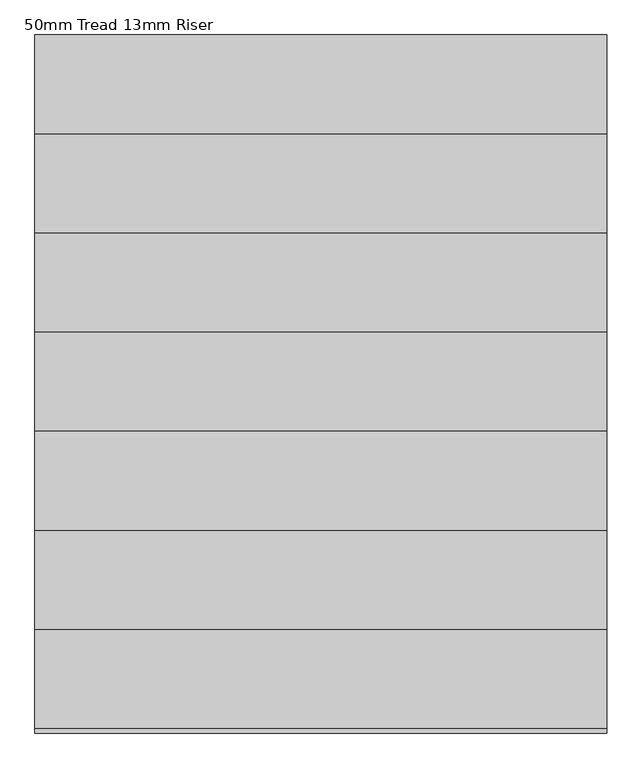
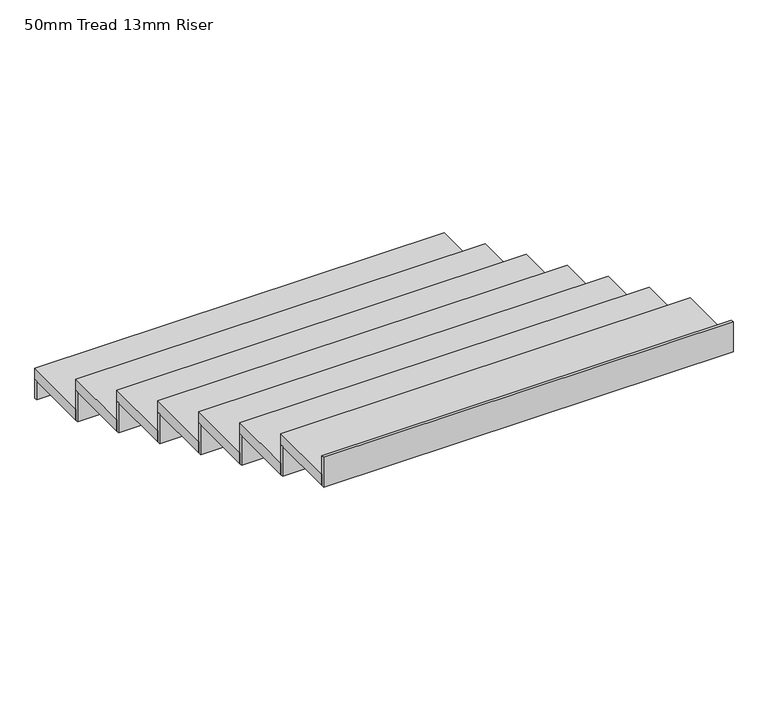
"""IFC4 building model written with IfcOpenShell, lengths in millimetres: stair flight geometry, 50mm Tread 13mm Riser."""

import ifcopenshell
import ifcopenshell.guid

model = None  # the IFC model being written
_history = None  # IfcOwnerHistory: only IFC2X3 demands one
_inside = {}  # id of a spatial element -> (the spatial element, [elements in it])
_under = {}  # id of a project, library or spatial element -> (it, [spatial elements below it])
_declared = {}  # id of a project -> (the project, [libraries it declares])
_typed = {}  # id of a type object -> (the type object, [elements of that type])
_made_of = {}  # id of a material, layer set ... -> (it, [elements and type objects made of it])


def new_model(schema):
    """Start an empty IFC model of exactly this schema.

    Asked for "IFC4X3", IfcOpenShell would pick the latest addendum, in which some entities
    have other attributes; the version numbers below select the first issue.
    IFC2X3 requires an IfcOwnerHistory on every rooted entity: one is made here for all.
    """
    global model, _history
    if schema == "IFC4X3":
        model = ifcopenshell.file(schema_version=(4, 3, 0, 0))
    else:
        model = ifcopenshell.file(schema=schema)
    _inside.clear()
    _under.clear()
    _declared.clear()
    _typed.clear()
    _made_of.clear()
    _history = None
    if model.schema == "IFC2X3":
        org = make("IfcOrganization", Name="unknown")
        user = make(
            "IfcPersonAndOrganization",
            ThePerson=make("IfcPerson", FamilyName="unknown"),
            TheOrganization=org,
        )
        app = make(
            "IfcApplication",
            ApplicationDeveloper=org,
            Version="unknown",
            ApplicationFullName="unknown",
            ApplicationIdentifier="unknown",
        )
        _history = make(
            "IfcOwnerHistory",
            OwningUser=user,
            OwningApplication=app,
            ChangeAction="ADDED",
            CreationDate=0,
        )
    return model


def make(cls, **values):
    """One entity of the class cls with the attributes given. An attribute that is None is left unset."""
    return model.create_entity(
        cls, **{name: value for name, value in values.items() if value is not None}
    )


def rooted(cls, **values):
    """An entity with a GlobalId (a new one), such as an element, a storey or a relation."""
    return make(cls, GlobalId=ifcopenshell.guid.new(), OwnerHistory=_history, **values)


def si_unit(unit_type, name, prefix=None):
    """IfcSIUnit, for example si_unit("LENGTHUNIT", "METRE", prefix="MILLI")."""
    return make("IfcSIUnit", UnitType=unit_type, Prefix=prefix, Name=name)


def assignment(units):
    """IfcUnitAssignment: the units of a project."""
    return None if units is None else make("IfcUnitAssignment", Units=units)


def point(xyz):
    """IfcCartesianPoint."""
    return None if xyz is None else make("IfcCartesianPoint", Coordinates=xyz)


def direction(xyz):
    """IfcDirection."""
    return None if xyz is None else make("IfcDirection", DirectionRatios=xyz)


def frame(location, z_axis=None, x_axis=None):
    """IfcAxis2Placement3D, a coordinate frame: its origin and axes. An axis left out is left unset."""
    return make(
        "IfcAxis2Placement3D",
        Location=point(location),
        Axis=direction(z_axis),
        RefDirection=direction(x_axis),
    )


def origin():
    """The frame at (0, 0, 0) with its axes left unset."""
    return frame((0.0, 0.0, 0.0))


def place(relative_to, where):
    """IfcLocalPlacement: puts the frame where relative to a parent placement (None: the world)."""
    return make(
        "IfcLocalPlacement", PlacementRelTo=relative_to, RelativePlacement=where
    )


def context(
    kind, dimensions, precision=None, world=None, true_north=None, identifier=None
):
    """IfcGeometricRepresentationContext, for example the 3D "Model" context."""
    return make(
        "IfcGeometricRepresentationContext",
        ContextIdentifier=identifier,
        ContextType=kind,
        CoordinateSpaceDimension=dimensions,
        Precision=precision,
        WorldCoordinateSystem=world,
        TrueNorth=true_north,
    )


def project(units=None, contexts=None):
    """IfcProject with its units and contexts."""
    return rooted(
        "IfcProject",
        Name="project",
        RepresentationContexts=contexts,
        UnitsInContext=assignment(units),
    )


def spatial(cls, under=None, at=None, **own):
    """A site, building, storey or space (cls), placed at a placement, below another one or the project."""
    s = rooted(cls, ObjectPlacement=at, **own)
    if under is not None:
        _under.setdefault(under.id(), (under, []))[1].append(s)
    return s


def polyline(points):
    """IfcPolyline through the points."""
    return make("IfcPolyline", Points=[point(p) for p in points])


def outline(outer, holes=None, kind="AREA"):
    """IfcArbitraryClosedProfileDef: a profile drawn as a closed curve; with holes, ...WithVoids."""
    if holes is None:
        return make("IfcArbitraryClosedProfileDef", ProfileType=kind, OuterCurve=outer)
    return make(
        "IfcArbitraryProfileDefWithVoids",
        ProfileType=kind,
        OuterCurve=outer,
        InnerCurves=holes,
    )


def extrude(swept, where, along, depth):
    """IfcExtrudedAreaSolid: the profile swept, set in the frame where, extruded along a direction by depth."""
    return make(
        "IfcExtrudedAreaSolid",
        SweptArea=swept,
        Position=where,
        ExtrudedDirection=direction(along),
        Depth=depth,
    )


def shape(context_of_items, identifier, shape_type, items):
    """IfcShapeRepresentation: the items that make up one representation, for example the "Body"."""
    return make(
        "IfcShapeRepresentation",
        ContextOfItems=context_of_items,
        RepresentationIdentifier=identifier,
        RepresentationType=shape_type,
        Items=items,
    )


def source(mapping_origin, context_of_items, identifier, shape_type, items):
    """IfcRepresentationMap: a shape defined once, which mapped items show again and again."""
    return make(
        "IfcRepresentationMap",
        MappingOrigin=mapping_origin,
        MappedRepresentation=shape(context_of_items, identifier, shape_type, items),
    )


def transform(
    local_origin,
    x_axis=None,
    y_axis=None,
    z_axis=None,
    scale=None,
    scale2=None,
    scale3=None,
    uniform=True,
):
    """IfcCartesianTransformationOperator3D, or its non-uniform kind. x_axis, y_axis, z_axis: its Axis1, 2, 3."""
    if uniform:
        return make(
            "IfcCartesianTransformationOperator3D",
            Axis1=direction(x_axis),
            Axis2=direction(y_axis),
            LocalOrigin=point(local_origin),
            Scale=scale,
            Axis3=direction(z_axis),
        )
    return make(
        "IfcCartesianTransformationOperator3DnonUniform",
        Axis1=direction(x_axis),
        Axis2=direction(y_axis),
        LocalOrigin=point(local_origin),
        Scale=scale,
        Axis3=direction(z_axis),
        Scale2=scale2,
        Scale3=scale3,
    )


def mapped(mapping_source, mapping_target):
    """IfcMappedItem: shows the shape of a source again, moved by a transform."""
    return make(
        "IfcMappedItem", MappingSource=mapping_source, MappingTarget=mapping_target
    )


def made_of(thing, what):
    """Note that an element or type object is made of a material, layer set ...; save() writes the relation."""
    if what is not None:
        _made_of.setdefault(what.id(), (what, []))[1].append(thing)
    return thing


def element(
    cls,
    number,
    at=None,
    inside=None,
    cuts=None,
    type_object=None,
    material=None,
    context=None,
    identifier="Body",
    shape_type=None,
    held_by="IfcProductDefinitionShape",
    body=None,
    shapes=None,
    **own,
):
    """One element of the class cls, such as IfcWall. Its Tag is "e" and its number.

    at: its placement. inside: the storey or other place that contains it. cuts: it is an
    opening in that element (IfcRelVoidsElement). A single representation is given by context,
    identifier, shape_type and body (its items); several are given by shapes. held_by: the class
    of the entity that holds the representations. save() writes the other relations.
    """
    e = rooted(cls, Tag="e%d" % number, ObjectPlacement=at, **own)
    if body is not None:
        shapes = [shape(context, identifier, shape_type, body)]
    if shapes is not None:
        e.Representation = make(held_by, Representations=shapes)
    if inside is not None:
        _inside.setdefault(inside.id(), (inside, []))[1].append(e)
    if cuts is not None:
        rooted(
            "IfcRelVoidsElement", RelatingBuildingElement=cuts, RelatedOpeningElement=e
        )
    if type_object is not None:
        _typed.setdefault(type_object.id(), (type_object, []))[1].append(e)
    return made_of(e, material)


def aggregate(whole, parts):
    """IfcRelAggregates: a whole, such as a stair, and the parts it consists of."""
    return rooted("IfcRelAggregates", RelatingObject=whole, RelatedObjects=parts)


def save(model, path):
    """Write the relations noted so far, then the file.

    IfcRelAggregates (storeys below a building ...), IfcRelContainedInSpatialStructure (elements
    in a storey), IfcRelDefinesByType, IfcRelAssociatesMaterial and IfcRelDeclares: one each for
    every whole, place, type object, material and project.
    """
    for whole, parts in _under.values():
        aggregate(whole, parts)
    for where, things in _inside.values():
        rooted(
            "IfcRelContainedInSpatialStructure",
            RelatedElements=things,
            RelatingStructure=where,
        )
    for kind, things in _typed.values():
        rooted("IfcRelDefinesByType", RelatedObjects=things, RelatingType=kind)
    for what, things in _made_of.values():
        rooted("IfcRelAssociatesMaterial", RelatedObjects=things, RelatingMaterial=what)
    for by, libraries in _declared.values():
        rooted("IfcRelDeclares", RelatingContext=by, RelatedDefinitions=libraries)
    model.write(path)


def stair_flight_50mm_tread_13mm_riser_d40b31cd(model_context):
    return source(origin(), model_context, "Body", "SweptSolid", [
        extrude(outline(polyline([(-13215.2814495, -5630.5731037), (-13215.2814495, -5618.0731037), (-11485.2814495, -5618.0731037), (-11485.2814495, -5630.5731037), (-13215.2814495, -5630.5731037)])), frame((0.0, 0.0, -1066.6666667), z_axis=(0.0, 0.0, 1.0), x_axis=(1.0, 0.0, 0.0)), (0.0, 0.0, 1.0), 83.3333333),
        extrude(outline(polyline([(-11485.2814495, -5918.0731037), (-13215.2814495, -5918.0731037), (-13215.2814495, -5618.0731037), (-11485.2814495, -5618.0731037), (-11485.2814495, -5918.0731037)])), frame((0.0, 0.0, -983.3333333), z_axis=(0.0, 0.0, 1.0), x_axis=(1.0, 0.0, 0.0)), (0.0, 0.0, 1.0), 50.0),
        extrude(outline(polyline([(-13215.2814495, -5930.5731037), (-13215.2814495, -5918.0731037), (-11485.2814495, -5918.0731037), (-11485.2814495, -5930.5731037), (-13215.2814495, -5930.5731037)])), frame((0.0, 0.0, -983.3333333), z_axis=(0.0, 0.0, 1.0), x_axis=(1.0, 0.0, 0.0)), (0.0, 0.0, 1.0), 133.3333333),
        extrude(outline(polyline([(-11485.2814495, -6218.0731037), (-13215.2814495, -6218.0731037), (-13215.2814495, -5918.0731037), (-11485.2814495, -5918.0731037), (-11485.2814495, -6218.0731037)])), frame((0.0, 0.0, -850.0), z_axis=(0.0, 0.0, 1.0), x_axis=(1.0, 0.0, 0.0)), (0.0, 0.0, 1.0), 50.0),
        extrude(outline(polyline([(-13215.2814495, -6230.5731037), (-13215.2814495, -6218.0731037), (-11485.2814495, -6218.0731037), (-11485.2814495, -6230.5731037), (-13215.2814495, -6230.5731037)])), frame((0.0, 0.0, -850.0), z_axis=(0.0, 0.0, 1.0), x_axis=(1.0, 0.0, 0.0)), (0.0, 0.0, 1.0), 133.3333333),
        extrude(outline(polyline([(-11485.2814495, -6518.0731037), (-13215.2814495, -6518.0731037), (-13215.2814495, -6218.0731037), (-11485.2814495, -6218.0731037), (-11485.2814495, -6518.0731037)])), frame((0.0, 0.0, -716.6666667), z_axis=(0.0, 0.0, 1.0), x_axis=(1.0, 0.0, 0.0)), (0.0, 0.0, 1.0), 50.0),
        extrude(outline(polyline([(-13215.2814495, -6530.5731037), (-13215.2814495, -6518.0731037), (-11485.2814495, -6518.0731037), (-11485.2814495, -6530.5731037), (-13215.2814495, -6530.5731037)])), frame((0.0, 0.0, -716.6666667), z_axis=(0.0, 0.0, 1.0), x_axis=(1.0, 0.0, 0.0)), (0.0, 0.0, 1.0), 133.3333333),
        extrude(outline(polyline([(-11485.2814495, -6818.0731037), (-13215.2814495, -6818.0731037), (-13215.2814495, -6518.0731037), (-11485.2814495, -6518.0731037), (-11485.2814495, -6818.0731037)])), frame((0.0, 0.0, -583.3333333), z_axis=(0.0, 0.0, 1.0), x_axis=(1.0, 0.0, 0.0)), (0.0, 0.0, 1.0), 50.0),
        extrude(outline(polyline([(-13215.2814495, -6830.5731037), (-13215.2814495, -6818.0731037), (-11485.2814495, -6818.0731037), (-11485.2814495, -6830.5731037), (-13215.2814495, -6830.5731037)])), frame((0.0, 0.0, -583.3333333), z_axis=(0.0, 0.0, 1.0), x_axis=(1.0, 0.0, 0.0)), (0.0, 0.0, 1.0), 133.3333333),
        extrude(outline(polyline([(-11485.2814495, -7118.0731037), (-13215.2814495, -7118.0731037), (-13215.2814495, -6818.0731037), (-11485.2814495, -6818.0731037), (-11485.2814495, -7118.0731037)])), frame((0.0, 0.0, -450.0), z_axis=(0.0, 0.0, 1.0), x_axis=(1.0, 0.0, 0.0)), (0.0, 0.0, 1.0), 50.0),
        extrude(outline(polyline([(-13215.2814495, -7130.5731037), (-13215.2814495, -7118.0731037), (-11485.2814495, -7118.0731037), (-11485.2814495, -7130.5731037), (-13215.2814495, -7130.5731037)])), frame((0.0, 0.0, -450.0), z_axis=(0.0, 0.0, 1.0), x_axis=(1.0, 0.0, 0.0)), (0.0, 0.0, 1.0), 133.3333333),
        extrude(outline(polyline([(-11485.2814495, -7418.0731037), (-13215.2814495, -7418.0731037), (-13215.2814495, -7118.0731037), (-11485.2814495, -7118.0731037), (-11485.2814495, -7418.0731037)])), frame((0.0, 0.0, -316.6666667), z_axis=(0.0, 0.0, 1.0), x_axis=(1.0, 0.0, 0.0)), (0.0, 0.0, 1.0), 50.0),
        extrude(outline(polyline([(-13215.2814495, -7430.5731037), (-13215.2814495, -7418.0731037), (-11485.2814495, -7418.0731037), (-11485.2814495, -7430.5731037), (-13215.2814495, -7430.5731037)])), frame((0.0, 0.0, -316.6666667), z_axis=(0.0, 0.0, 1.0), x_axis=(1.0, 0.0, 0.0)), (0.0, 0.0, 1.0), 133.3333333),
        extrude(outline(polyline([(-13215.2814495, -7730.5731037), (-13215.2814495, -7718.0731037), (-11485.2814495, -7718.0731037), (-11485.2814495, -7730.5731037), (-13215.2814495, -7730.5731037)])), frame((0.0, 0.0, -183.3333333), z_axis=(0.0, 0.0, 1.0), x_axis=(1.0, 0.0, 0.0)), (0.0, 0.0, 1.0), 133.3333333),
        extrude(outline(polyline([(-11485.2814495, -7718.0731037), (-13215.2814495, -7718.0731037), (-13215.2814495, -7418.0731037), (-11485.2814495, -7418.0731037), (-11485.2814495, -7718.0731037)])), frame((0.0, 0.0, -183.3333333), z_axis=(0.0, 0.0, 1.0), x_axis=(1.0, 0.0, 0.0)), (0.0, 0.0, 1.0), 50.0),
    ])


if __name__ == "__main__":
    model = new_model("IFC4")
    model_context = context("Model", 3, world=origin())
    ifc_project = project(units=[si_unit("LENGTHUNIT", "METRE", prefix="MILLI")], contexts=[model_context])
    site = spatial("IfcSite", under=ifc_project)
    building = spatial("IfcBuilding", under=site)
    placement = place(None, origin())
    stair_flight_50mm_tread_13mm_riser_shape = stair_flight_50mm_tread_13mm_riser_d40b31cd(model_context)
    element("IfcStairFlight", 1, ObjectType="50mm Tread 13mm Riser", at=placement, inside=building, context=model_context, shape_type="MappedRepresentation", body=[
        mapped(stair_flight_50mm_tread_13mm_riser_shape, transform((0.0, 0.0, 0.0), x_axis=(1.0, 0.0, 0.0), y_axis=(0.0, 1.0, 0.0), z_axis=(0.0, 0.0, 1.0))),
    ])
    save(model, "model.ifc")
